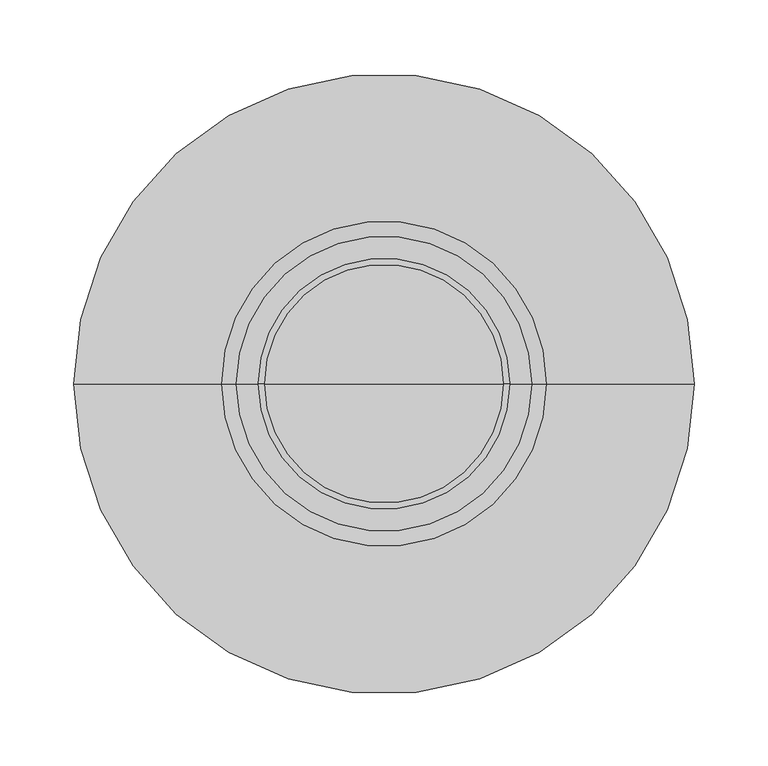
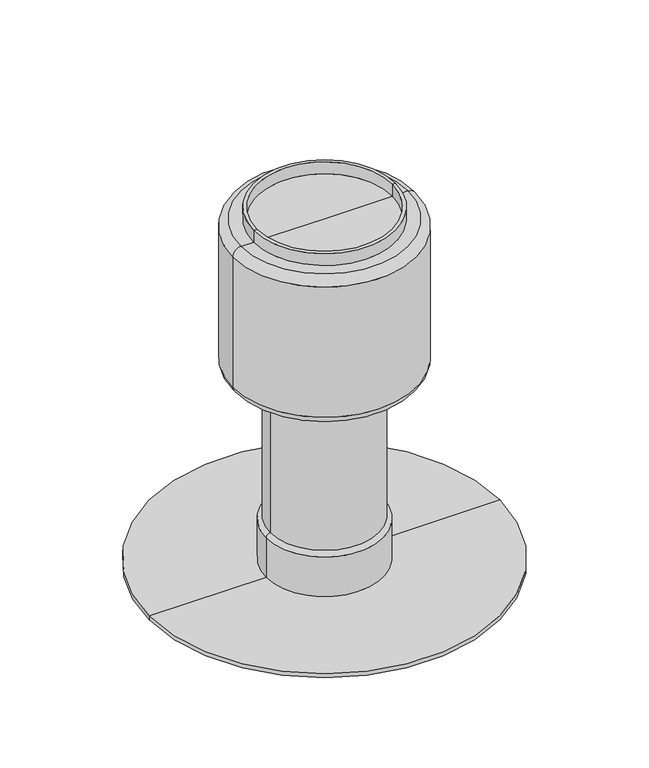
"""IFC4 building model written with IfcOpenShell, lengths in millimetres: proxy geometry, TN_Кровельный вакуумный аэратор : Кровельный вакуумный аэратор с клапаном 450x420 мм."""

from ifc_helpers import new_model, si_unit, point, frame, origin, place, context, project, spatial, polyline, circle_curve, ellipse_curve, trimmed, source, transform, mapped, element, save
from ifc_brep_helpers import plane_surface, cylinder_surface, revolved_surface, advanced_brep


def specialty_equipment_0526c882(model_context):
    return source(origin(), model_context, "Body", "AdvancedBrep", [
        advanced_brep(
        [(81.0, 0.0, 435.0), (-81.0, 0.0, 435.0), (0.0, 0.0, 435.0), (81.0, 0.0, 450.0), (-81.0, 0.0, 450.0), (85.0, 0.0, 450.0), (-85.0, 0.0, 450.0), (85.0, 0.0, 435.0), (-85.0, 0.0, 435.0), (100.0, 0.0, 435.0), (-100.0, 0.0, 435.0), (110.0, 0.0, 425.0), (-110.0, 0.0, 425.0), (110.0, 0.0, 260.0), (-110.0, 0.0, 260.0), (100.0, 0.0, 250.0), (-100.0, 0.0, 250.0), (65.0, 0.0, 250.0), (-65.0, 0.0, 250.0), (65.0, 0.0, 60.0), (-65.0, 0.0, 60.0), (70.0, 0.0, 55.0), (-70.0, 0.0, 55.0), (70.0, 0.0, 5.0), (-70.0, 0.0, 5.0), (210.0, 0.0, 5.0), (-210.0, 0.0, 5.0), (210.0, 0.0, 0.0), (-210.0, 0.0, 0.0), (0.0, 0.0, 0.0)],
        [
            (0, 1, circle_curve(frame((0.0, 0.0, 435.0), z_axis=(0.0, 0.0, 1.0), x_axis=(-1.0, 0.0, 0.0)), 81.0)),
            (1, 2),
            (2, 0),
            (1, 0, circle_curve(frame((0.0, 0.0, 435.0), z_axis=(0.0, 0.0, 1.0), x_axis=(-1.0, 0.0, 0.0)), 81.0)),
            (3, 4, circle_curve(frame((0.0, 0.0, 450.0), z_axis=(0.0, 0.0, 1.0), x_axis=(-1.0, 0.0, 0.0)), 81.0)),
            (4, 1),
            (0, 3),
            (4, 3, circle_curve(frame((0.0, 0.0, 450.0), z_axis=(0.0, 0.0, 1.0), x_axis=(-1.0, 0.0, 0.0)), 81.0)),
            (5, 6, circle_curve(frame((0.0, 0.0, 450.0), z_axis=(0.0, 0.0, 1.0), x_axis=(-1.0, 0.0, 0.0)), 85.0)),
            (6, 4),
            (3, 5),
            (6, 5, circle_curve(frame((0.0, 0.0, 450.0), z_axis=(0.0, 0.0, 1.0), x_axis=(-1.0, 0.0, 0.0)), 85.0)),
            (7, 8, circle_curve(frame((0.0, 0.0, 435.0), z_axis=(0.0, 0.0, 1.0), x_axis=(-1.0, 0.0, 0.0)), 85.0)),
            (8, 6),
            (5, 7),
            (8, 7, circle_curve(frame((0.0, 0.0, 435.0), z_axis=(0.0, 0.0, 1.0), x_axis=(-1.0, 0.0, 0.0)), 85.0)),
            (9, 10, circle_curve(frame((0.0, 0.0, 435.0), z_axis=(0.0, 0.0, 1.0), x_axis=(-1.0, 0.0, 0.0)), 100.0)),
            (10, 8),
            (7, 9),
            (10, 9, circle_curve(frame((0.0, 0.0, 435.0), z_axis=(0.0, 0.0, 1.0), x_axis=(-1.0, 0.0, 0.0)), 100.0)),
            (11, 12, circle_curve(frame((0.0, 0.0, 425.0), z_axis=(0.0, 0.0, 1.0), x_axis=(-1.0, 0.0, 0.0)), 110.0)),
            (12, 10, circle_curve(frame((-100.0, 0.0, 425.0), z_axis=(0.0, 1.0, 0.0), x_axis=(1.0, 0.0, 0.0)), 10.0)),
            (9, 11, circle_curve(frame((100.0, 0.0, 425.0), z_axis=(0.0, 1.0, 0.0), x_axis=(-1.0, 0.0, 0.0)), 10.0)),
            (12, 11, circle_curve(frame((0.0, 0.0, 425.0), z_axis=(0.0, 0.0, 1.0), x_axis=(-1.0, 0.0, 0.0)), 110.0)),
            (13, 14, circle_curve(frame((0.0, 0.0, 260.0), z_axis=(0.0, 0.0, 1.0), x_axis=(-1.0, 0.0, 0.0)), 110.0)),
            (14, 12),
            (11, 13),
            (14, 13, circle_curve(frame((0.0, 0.0, 260.0), z_axis=(0.0, 0.0, 1.0), x_axis=(-1.0, 0.0, 0.0)), 110.0)),
            (15, 16, circle_curve(frame((0.0, 0.0, 250.0), z_axis=(0.0, 0.0, 1.0), x_axis=(-1.0, 0.0, 0.0)), 100.0)),
            (16, 14, circle_curve(frame((-100.0, 0.0, 260.0), z_axis=(0.0, 1.0, 0.0), x_axis=(1.0, 0.0, 0.0)), 10.0)),
            (13, 15, circle_curve(frame((100.0, 0.0, 260.0), z_axis=(0.0, 1.0, 0.0), x_axis=(-1.0, 0.0, 0.0)), 10.0)),
            (16, 15, circle_curve(frame((0.0, 0.0, 250.0), z_axis=(0.0, 0.0, 1.0), x_axis=(-1.0, 0.0, 0.0)), 100.0)),
            (17, 18, circle_curve(frame((0.0, 0.0, 250.0), z_axis=(0.0, 0.0, 1.0), x_axis=(-1.0, 0.0, 0.0)), 65.0)),
            (18, 16),
            (15, 17),
            (18, 17, circle_curve(frame((0.0, 0.0, 250.0), z_axis=(0.0, 0.0, 1.0), x_axis=(-1.0, 0.0, 0.0)), 65.0)),
            (19, 20, circle_curve(frame((0.0, 0.0, 60.0), z_axis=(0.0, 0.0, 1.0), x_axis=(-1.0, 0.0, 0.0)), 65.0)),
            (20, 18),
            (17, 19),
            (20, 19, circle_curve(frame((0.0, 0.0, 60.0), z_axis=(0.0, 0.0, 1.0), x_axis=(-1.0, 0.0, 0.0)), 65.0)),
            (21, 22, circle_curve(frame((0.0, 0.0, 55.0), z_axis=(0.0, 0.0, 1.0), x_axis=(-1.0, 0.0, 0.0)), 70.0)),
            (22, 20, circle_curve(frame((-65.0, 0.0, 55.0), z_axis=(0.0, 1.0, 0.0), x_axis=(1.0, 0.0, 0.0)), 5.0)),
            (19, 21, circle_curve(frame((65.0, 0.0, 55.0), z_axis=(0.0, 1.0, 0.0), x_axis=(-1.0, 0.0, 0.0)), 5.0)),
            (22, 21, circle_curve(frame((0.0, 0.0, 55.0), z_axis=(0.0, 0.0, 1.0), x_axis=(-1.0, 0.0, 0.0)), 70.0)),
            (23, 24, circle_curve(frame((0.0, 0.0, 5.0), z_axis=(0.0, 0.0, 1.0), x_axis=(-1.0, 0.0, 0.0)), 70.0)),
            (24, 22),
            (21, 23),
            (24, 23, circle_curve(frame((0.0, 0.0, 5.0), z_axis=(0.0, 0.0, 1.0), x_axis=(-1.0, 0.0, 0.0)), 70.0)),
            (25, 26, circle_curve(frame((0.0, 0.0, 5.0), z_axis=(0.0, 0.0, 1.0), x_axis=(-1.0, 0.0, 0.0)), 210.0)),
            (26, 24),
            (23, 25),
            (26, 25, circle_curve(frame((0.0, 0.0, 5.0), z_axis=(0.0, 0.0, 1.0), x_axis=(-1.0, 0.0, 0.0)), 210.0)),
            (27, 28, circle_curve(frame((0.0, 0.0, 0.0), z_axis=(0.0, 0.0, 1.0), x_axis=(-1.0, 0.0, 0.0)), 210.0)),
            (28, 26),
            (25, 27),
            (28, 27, circle_curve(frame((0.0, 0.0, 0.0), z_axis=(0.0, 0.0, 1.0), x_axis=(-1.0, 0.0, 0.0)), 210.0)),
            (29, 28),
            (27, 29),
        ],
        [
            plane_surface(frame((0.0, 0.0, 435.0), z_axis=(0.0, 0.0, 1.0), x_axis=(-1.0, 0.0, 0.0))),
            revolved_surface(polyline([(-81.0, 0.0, 435.0), (-81.0, 0.0, 450.0)]), (0.0, 0.0, 450.0), (0.0, 0.0, -1.0)),
            plane_surface(frame((0.0, 0.0, 450.0), z_axis=(0.0, 0.0, 1.0), x_axis=(-1.0, 0.0, 0.0))),
            cylinder_surface(frame((0.0, 0.0, 450.0), z_axis=(0.0, 0.0, -1.0), x_axis=(-1.0, 0.0, 0.0)), 85.0),
            revolved_surface(trimmed(ellipse_curve(frame((-100.0, 0.0, 425.0), z_axis=(0.0, -1.0, 0.0), x_axis=(1.0, 0.0, 0.0)), 10.0, 10.0), [point((-100.0, 0.0, 435.0))], [point((-110.0, 0.0, 425.0))], True, "CARTESIAN"), (0.0, 0.0, 450.0), (0.0, 0.0, -1.0)),
            cylinder_surface(frame((0.0, 0.0, 450.0), z_axis=(0.0, 0.0, -1.0), x_axis=(-1.0, 0.0, 0.0)), 110.0),
            revolved_surface(trimmed(ellipse_curve(frame((-100.0, 0.0, 260.0), z_axis=(0.0, -1.0, 0.0), x_axis=(1.0, 0.0, 0.0)), 10.0, 10.0), [point((-110.0, 0.0, 260.0))], [point((-100.0, 0.0, 250.0))], True, "CARTESIAN"), (0.0, 0.0, 450.0), (0.0, 0.0, -1.0)),
            plane_surface(frame((0.0, 0.0, 250.0), z_axis=(0.0, 0.0, -1.0), x_axis=(-1.0, 0.0, 0.0))),
            cylinder_surface(frame((0.0, 0.0, 450.0), z_axis=(0.0, 0.0, -1.0), x_axis=(-1.0, 0.0, 0.0)), 65.0),
            revolved_surface(trimmed(ellipse_curve(frame((-65.0, 0.0, 55.0), z_axis=(0.0, -1.0, 0.0), x_axis=(1.0, 0.0, 0.0)), 5.0, 5.0), [point((-65.0, 0.0, 60.0))], [point((-70.0, 0.0, 55.0))], True, "CARTESIAN"), (0.0, 0.0, 450.0), (0.0, 0.0, -1.0)),
            cylinder_surface(frame((0.0, 0.0, 450.0), z_axis=(0.0, 0.0, -1.0), x_axis=(-1.0, 0.0, 0.0)), 70.0),
            plane_surface(frame((0.0, 0.0, 5.0), z_axis=(0.0, 0.0, 1.0), x_axis=(-1.0, 0.0, 0.0))),
            cylinder_surface(frame((0.0, 0.0, 450.0), z_axis=(0.0, 0.0, -1.0), x_axis=(-1.0, 0.0, 0.0)), 210.0),
            plane_surface(frame((0.0, 0.0, 0.0), z_axis=(0.0, 0.0, -1.0), x_axis=(-1.0, 0.0, 0.0))),
        ],
        [
            (0, [[1, 2, 3]]),
            (0, [[4, -3, -2]]),
            (1, [[5, 6, -1, 7]]),
            (1, [[8, -7, -4, -6]]),
            (2, [[9, 10, -5, 11]]),
            (2, [[12, -11, -8, -10]]),
            (3, [[13, 14, -9, 15]]),
            (3, [[16, -15, -12, -14]]),
            (0, [[17, 18, -13, 19]]),
            (0, [[20, -19, -16, -18]]),
            (4, [[21, 22, -17, 23]]),
            (4, [[24, -23, -20, -22]]),
            (5, [[25, 26, -21, 27]]),
            (5, [[28, -27, -24, -26]]),
            (6, [[29, 30, -25, 31]]),
            (6, [[32, -31, -28, -30]]),
            (7, [[33, 34, -29, 35]]),
            (7, [[36, -35, -32, -34]]),
            (8, [[37, 38, -33, 39]]),
            (8, [[40, -39, -36, -38]]),
            (9, [[41, 42, -37, 43]]),
            (9, [[44, -43, -40, -42]]),
            (10, [[45, 46, -41, 47]]),
            (10, [[48, -47, -44, -46]]),
            (11, [[49, 50, -45, 51]]),
            (11, [[52, -51, -48, -50]]),
            (12, [[53, 54, -49, 55]]),
            (12, [[56, -55, -52, -54]]),
            (13, [[57, -53, 58]]),
            (13, [[-58, -56, -57]]),
        ],
    ),
    ])


if __name__ == "__main__":
    model = new_model("IFC4")
    model_context = context("Model", 3, world=origin())
    ifc_project = project(units=[si_unit("LENGTHUNIT", "METRE", prefix="MILLI")], contexts=[model_context])
    site = spatial("IfcSite", under=ifc_project)
    building = spatial("IfcBuilding", under=site)
    placement = place(None, origin())
    specialty_equipment_shape = specialty_equipment_0526c882(model_context)
    element("IfcBuildingElementProxy", 1, Name="TN_Кровельный вакуумный аэратор : Кровельный вакуумный аэратор с клапаном 450x420 мм", ObjectType="TN_Кровельный вакуумный аэратор : Кровельный вакуумный аэратор с клапаном 450x420 мм", at=placement, inside=building, context=model_context, shape_type="MappedRepresentation", body=[
        mapped(specialty_equipment_shape, transform((0.0, 0.0, 0.0), x_axis=(1.0, 0.0, 0.0), y_axis=(0.0, 1.0, 0.0), z_axis=(0.0, 0.0, 1.0))),
    ])
    save(model, "model.ifc")

# Revit data of these elements
# Type "TN_Кровельный вакуумный аэратор : Кровельный вакуумный аэратор с клапаном 450x420 мм"
#   ADSK_Группирование = "Комплектующие и воронки"
#   Description = "Кровельный вакуумный аэратор ТехноНИКОЛЬ с клапаном 450x420 мм.\r\nВакуумный аэратор изготовлен из полипропилена. Изделие используется на «дышащих» кровлях и для санации. Служит для снижения отрывной силы и уменьшения риска срыва кровельного покрытия. Благодаря своим характеристикам аэратор может использоваться в зонах сильного или даже аномального ветра. Но установка вакуумного аэратора не заменяет механического крепления кровельного материала."
#   Manufacturer = "ТехноНИКОЛЬ"
#   URL = "https://shop.tn.ru/krovel-nyj-vakuumnyj-ajerator-s-klapanom-450x420-mm"
#   ADSK_Примечание = ""
#   ADSK_Обозначение = "ТехноНИКОЛЬ"
#   ADSK_Наименование = "Кровельный вакуумный аэратор с клапаном 450x420 мм"
#   ADSK_Марка = ""
#   ADSK_Код изделия = "472155"
#   ADSK_Завод-изготовитель = "ТехноНИКОЛЬ"
#   ADSK_Единица измерения = "шт."
#   ADSK_Группирование = "Комплектующие и воронки"
#   ADSK_URL страницы изделия = "https://shop.tn.ru/krovel-nyj-vakuumnyj-ajerator-s-klapanom-450x420-mm"
#   ADSK_URL документации изделия = ""
#   Default Elevation = 1219.2 mm
#   ADSK_Масса = 1.2
#   ADSK_Количество = 1
#   Материал = TN_ПВХ_Черный
# Element 1 (IfcBuildingElementProxy, "TN_Кровельный вакуумный аэратор : Кровельный вакуумный аэратор с клапаном 450x420 мм")
#   Materials on its faces: "TN_ПВХ_Черный"
# Materials
#   "TN_ПВХ_Черный": class "Типовые", colour RGB 48 48 48, transparency 0, Cost = 0
